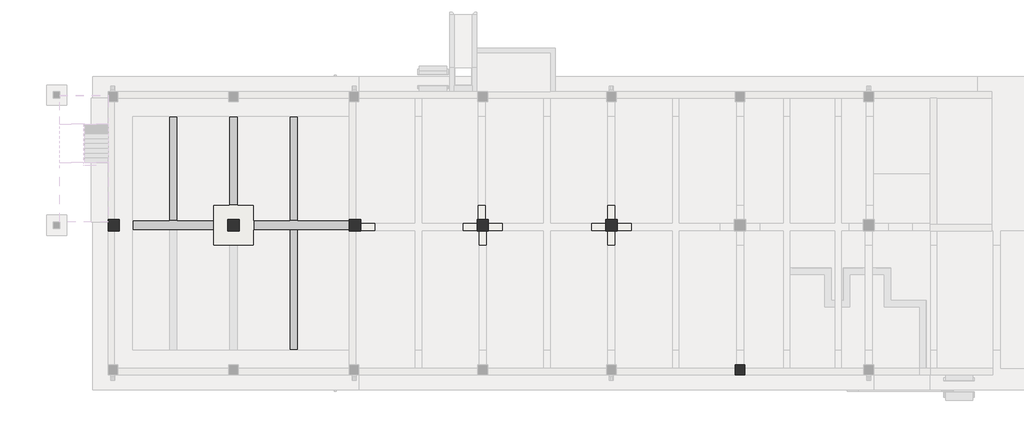
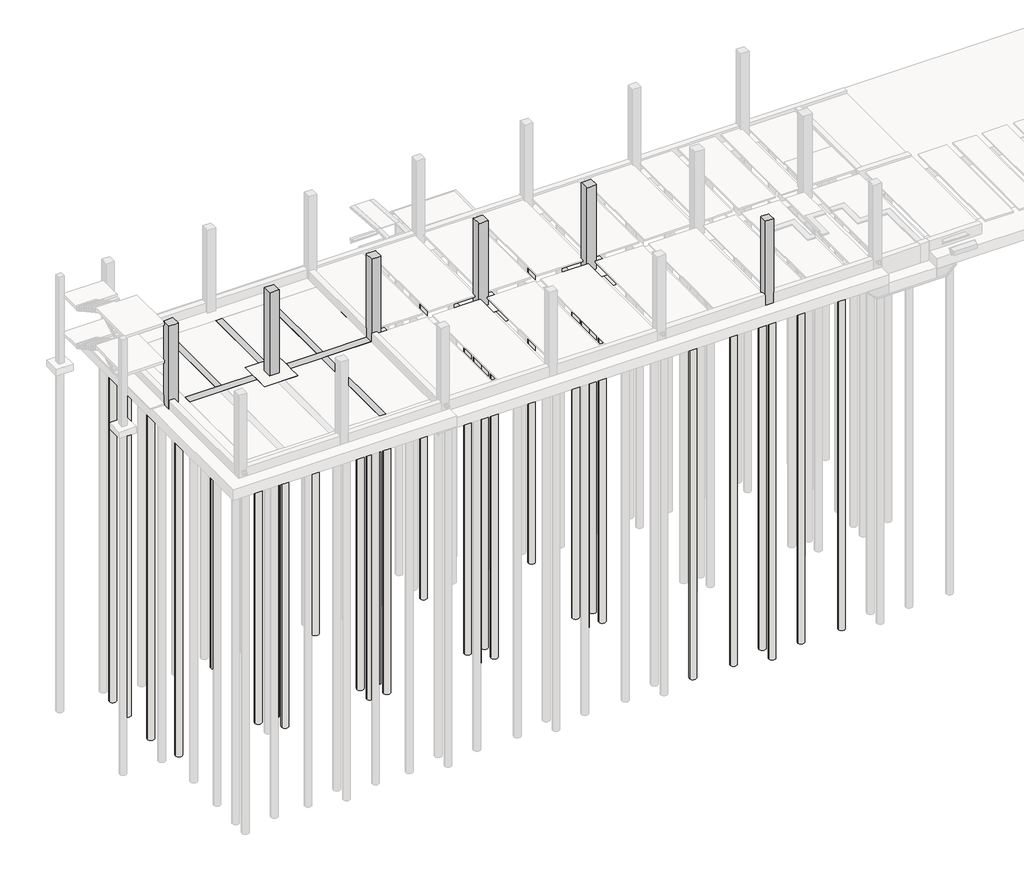
# One storey, part 4 of 7: 33 slabs, 8 beams, 6 columns.
"""IFC4 building model written with IfcOpenShell, lengths in millimetres."""

from ifc_helpers import new_model, si_unit, point, frame, frame_2d, origin, place, context, project, spatial, polyline, circle_curve, trimmed, segment, composite_curve, outline, extrude, faceted_brep, element, save

model = new_model("IFC4")

# Units and contexts
model_context = context("Model", 3, world=origin())
ifc_project = project(units=[si_unit("LENGTHUNIT", "METRE", prefix="MILLI")], contexts=[model_context])

# Site, building, storey
site = spatial("IfcSite", under=ifc_project)
building = spatial("IfcBuilding", under=site)
storey = spatial("IfcBuildingStorey", under=building, Name="H.P.P", Elevation=4500.0)

# Beams
placement = place(None, origin())
element("IfcBeam", 1, ObjectType="RC Beam_Rectangular : H_SB_AR S16_TG-UG_500x700_FB1A", at=placement, inside=storey, context=model_context, shape_type="Brep", body=[
    faceted_brep([(11000.0, -15750.0, 3400.0), (11500.0, -15750.0, 3400.0), (11500.0, -15750.0, 3840.0), (11500.0, -15750.0, 3950.0), (11500.0, -15750.0, 4100.0), (11000.0, -15750.0, 4100.0), (11000.0, -15750.0, 3950.0), (11000.0, -15750.0, 3840.0), (11500.0, -8299.9999999, 4100.0), (11000.0, -8299.9999999, 4100.0), (11500.0, -8299.9999999, 3950.0), (11500.0, -8299.9999999, 3400.0), (11500.0, -8299.9999999, 3840.0), (11000.0, -8299.9999999, 3400.0), (11000.0, -8299.9999999, 3950.0), (11000.0, -8299.9999999, 3840.0)], [[[0, 1, 2, 3, 4, 5, 6, 7]], [[5, 4, 8, 9]], [[10, 8, 4, 3, 2, 1, 11, 12]], [[1, 0, 13, 11]], [[9, 14, 15, 13, 0, 7, 6, 5]], [[9, 8, 10, 12, 11, 13, 15, 14]]]),
])
element("IfcBeam", 2, ObjectType="RC Beam_Rectangular : H_SB_AR S16_TG-UG_600x800_FG2", at=placement, inside=storey, context=model_context, shape_type="Brep", body=[
    faceted_brep([(6250.0000003, -7700.0, 4100.0), (6250.0000003, -8300.0, 4100.0), (6250.0000003, -8300.0, 3950.0), (6250.0000003, -8300.0, 3840.0), (6250.0000003, -8300.0, 3300.0), (6250.0000003, -7700.0, 3300.0), (6250.0000003, -7700.0, 3840.0), (6250.0000003, -7700.0, 3950.0), (1250.0000003, -7700.0, 3300.0), (1250.0000003, -8300.0, 3300.0), (1250.0000003, -8300.0, 3840.0), (1250.0000003, -8300.0, 3950.0), (1250.0000003, -8300.0, 4100.0), (1250.0000003, -7700.0, 4100.0), (1250.0000003, -7700.0, 3950.0), (1250.0000003, -7700.0, 3840.0), (4000.0, -7700.0, 4100.0), (3500.0, -7700.0, 4100.0), (3500.0, -8300.0, 4100.0), (4000.0, -8300.0, 4100.0)], [[[0, 1, 2, 3, 4, 5, 6, 7]], [[8, 9, 10, 11, 12, 13, 14, 15]], [[1, 0, 16, 17, 13, 12, 18, 19]], [[9, 4, 3, 2, 1, 19, 18, 12, 11, 10]], [[5, 4, 9, 8]], [[5, 8, 15, 14, 13, 17, 16, 0, 7, 6]]]),
])
element("IfcBeam", 3, ObjectType="RC Beam_Rectangular : H_SB_AR S16_TG-UG_600x800_FG2", at=placement, inside=storey, context=model_context, shape_type="Brep", body=[
    faceted_brep([(8750.0000003, -7699.9999999, 3300.0), (8750.0000003, -8299.9999999, 3300.0), (8750.0000003, -8299.9999999, 3840.0), (8750.0000003, -8299.9999999, 3950.0), (8750.0000003, -8299.9999999, 4100.0), (8750.0000003, -7699.9999999, 4100.0), (8750.0000003, -7699.9999999, 3950.0), (8750.0000003, -7699.9999999, 3840.0), (11000.0, -8299.9999999, 4100.0), (11500.0, -8299.9999999, 4100.0), (14700.0000001, -8299.9999999, 4100.0), (14700.0000001, -7699.9999999, 4100.0), (11500.0, -7699.9999999, 4100.0), (11000.0, -7699.9999999, 4100.0), (13800.0000001, -8299.9999999, 4000.0), (14700.0000001, -8299.9999999, 4000.0), (13800.0000001, -8299.9999999, 3300.0), (13800.0000001, -8299.9999999, 3840.0), (13800.0000001, -8299.9999999, 3950.0), (13800.0000001, -7699.9999999, 3300.0), (14700.0000001, -7699.9999999, 4000.0), (13800.0000001, -7699.9999999, 4000.0), (13800.0000001, -7699.9999999, 3950.0), (13800.0000001, -7699.9999999, 3840.0)], [[[0, 1, 2, 3, 4, 5, 6, 7]], [[5, 4, 8, 9, 10, 11, 12, 13]], [[14, 15, 10, 9, 8, 4, 3, 2, 1, 16, 17, 18]], [[1, 0, 19, 16]], [[20, 21, 22, 23, 19, 0, 7, 6, 5, 13, 12, 11]], [[14, 21, 20, 15]], [[21, 14, 18, 17, 16, 19, 23, 22]], [[11, 10, 15, 20]]]),
])
element("IfcBeam", 4, ObjectType="RC Beam_Rectangular : H_SB_AR S16_TG-UG_500x700_FG1", at=placement, inside=storey, context=model_context, shape_type="Brep", body=[
    faceted_brep([(14700.0, -15750.0, 4100.0), (14700.0, -15750.0, 3950.0), (14700.0, -15750.0, 3840.0), (14700.0, -15750.0, 3400.0), (15200.0, -15750.0, 3400.0), (15200.0, -15750.0, 4100.0), (15200.0, -8350.0, 4100.0), (15100.0, -8350.0, 4100.0), (14700.0, -8350.0, 4100.0), (15200.0, -9250.0, 3400.0), (15200.0, -9250.0, 4000.0), (15200.0, -8350.0, 4000.0), (14700.0, -9250.0, 3400.0), (14700.0, -8350.0, 4000.0), (14700.0, -9250.0, 4000.0), (14700.0, -9250.0, 3950.0), (14700.0, -9250.0, 3840.0)], [[[0, 1, 2, 3, 4, 5]], [[0, 5, 6, 7, 8]], [[5, 4, 9, 10, 11, 6]], [[4, 3, 12, 9]], [[3, 2, 1, 0, 8, 13, 14, 15, 16, 12]], [[10, 14, 13, 11]], [[14, 10, 9, 12, 16, 15]], [[8, 7, 6, 11, 13]]]),
])
element("IfcBeam", 5, ObjectType="RC Beam_Rectangular : H_SB_AR S16_TG-UG_500x700_FB1A", at=placement, inside=storey, context=model_context, shape_type="Brep", body=[
    faceted_brep([(4000.0, -1250.0000001, 3400.0), (3500.0, -1250.0000001, 3400.0), (3500.0, -1250.0000001, 3840.0), (3500.0, -1250.0000001, 3950.0), (3500.0, -1250.0000001, 4100.0), (4000.0, -1250.0000001, 4100.0), (4000.0, -1250.0000001, 3950.0), (4000.0, -1250.0000001, 3840.0), (3500.0, -7700.0, 4100.0), (4000.0, -7700.0, 4100.0), (4000.0, -7700.0, 3950.0), (4000.0, -7700.0, 3840.0), (4000.0, -7700.0, 3400.0), (3500.0, -7700.0, 3400.0), (3500.0, -7700.0, 3840.0), (3500.0, -7700.0, 3950.0)], [[[0, 1, 2, 3, 4, 5, 6, 7]], [[5, 4, 8, 9]], [[5, 9, 10, 11, 12, 0, 7, 6]], [[1, 0, 12, 13]], [[8, 4, 3, 2, 1, 13, 14, 15]], [[9, 8, 15, 14, 13, 12, 11, 10]]]),
])
element("IfcBeam", 6, ObjectType="RC Beam_Rectangular : H_SB_AR S16_TG-UG_500x700_FG1", at=placement, inside=storey, context=model_context, shape_type="Brep", body=[
    faceted_brep([(7750.0, -6750.0000001, 4100.0), (7250.0, -6750.0000001, 4100.0), (7250.0, -6750.0000001, 3950.0), (7250.0, -6750.0000001, 3840.0), (7250.0, -6750.0000001, 3400.0), (7750.0, -6750.0000001, 3400.0), (7750.0, -6750.0000001, 3840.0), (7750.0, -6750.0000001, 3950.0), (7750.0, -1250.0000001, 3400.0), (7250.0, -1250.0000001, 3400.0), (7250.0, -1250.0000001, 3840.0), (7250.0, -1250.0000001, 3950.0), (7250.0, -1250.0000001, 4100.0), (7750.0, -1250.0000001, 4100.0), (7750.0, -1250.0000001, 3950.0), (7750.0, -1250.0000001, 3840.0)], [[[0, 1, 2, 3, 4, 5, 6, 7]], [[8, 9, 10, 11, 12, 13, 14, 15]], [[1, 0, 13, 12]], [[13, 0, 7, 6, 5, 8, 15, 14]], [[5, 4, 9, 8]], [[1, 12, 11, 10, 9, 4, 3, 2]]]),
])
element("IfcBeam", 7, ObjectType="RC Beam_Rectangular : H_SB_AR S16_TG-UG_500x700_FB1A", at=placement, inside=storey, context=model_context, shape_type="Brep", body=[
    faceted_brep([(11500.0, -1250.0000001, 3400.0), (11000.0, -1250.0000001, 3400.0), (11000.0, -1250.0000001, 3840.0), (11000.0, -1250.0000001, 3950.0), (11000.0, -1250.0000001, 4100.0), (11500.0, -1250.0000001, 4100.0), (11500.0, -1250.0000001, 3950.0), (11500.0, -1250.0000001, 3840.0), (11000.0, -7699.9999999, 4100.0), (11500.0, -7699.9999999, 4100.0), (11500.0, -7699.9999999, 3950.0), (11500.0, -7699.9999999, 3840.0), (11500.0, -7699.9999999, 3400.0), (11000.0, -7699.9999999, 3400.0), (11000.0, -7699.9999999, 3840.0), (11000.0, -7699.9999999, 3950.0)], [[[0, 1, 2, 3, 4, 5, 6, 7]], [[5, 4, 8, 9]], [[5, 9, 10, 11, 12, 0, 7, 6]], [[1, 0, 12, 13]], [[8, 4, 3, 2, 1, 13, 14, 15]], [[9, 8, 15, 14, 13, 12, 11, 10]]]),
])
element("IfcBeam", 8, ObjectType="RC Beam_Rectangular : H_SB_AR S16_TG-UG_500x700_FG1", at=placement, inside=storey, context=model_context, shape_type="Brep", body=[
    faceted_brep([(14700.0, -1250.0000001, 3400.0), (14700.0, -1250.0000001, 3840.0), (14700.0, -1250.0000001, 3950.0), (14700.0, -1250.0000001, 4100.0), (15200.0, -1250.0000001, 4100.0), (15200.0, -1250.0000001, 3400.0), (14700.0, -7650.0, 4100.0), (15100.0, -7650.0, 4100.0), (15200.0, -7650.0, 4100.0), (15200.0, -7650.0, 4000.0), (15200.0, -6750.0, 4000.0), (15200.0, -6750.0, 3400.0), (14700.0, -6750.0, 3400.0), (14700.0, -6750.0, 3840.0), (14700.0, -6750.0, 3950.0), (14700.0, -6750.0, 4000.0), (14700.0, -7650.0, 4000.0)], [[[0, 1, 2, 3, 4, 5]], [[4, 3, 6, 7, 8]], [[5, 4, 8, 9, 10, 11]], [[0, 5, 11, 12]], [[3, 2, 1, 0, 12, 13, 14, 15, 16, 6]], [[15, 10, 9, 16]], [[10, 15, 14, 13, 12, 11]], [[8, 7, 6, 16, 9]]]),
])

# Columns
element("IfcColumn", 9, ObjectType="RC_Column_Rectangular : H_SC_AR S15_RC Col-AG_700x700_C1", at=placement, inside=storey, context=model_context, shape_type="Brep", body=[
    faceted_brep([(400.0, -7650.0, 4100.0), (400.0, -8350.0, 4100.0), (100.0, -8350.0, 4100.0), (-300.0, -8350.0, 4100.0), (-300.0, -7650.0, 4100.0), (100.0, -7650.0, 4100.0), (400.0, -7650.0, 10450.0), (400.0, -7700.0, 10450.0), (400.0, -7700.0, 10600.0), (400.0, -8300.0, 10600.0), (400.0, -8300.0, 10450.0), (400.0, -8350.0, 10450.0), (399.4974747, -8350.0, 10450.0), (399.4974747, -8350.0, 10600.0), (100.0, -8350.0, 10600.0), (-300.0, -8350.0, 10600.0), (-300.0, -8350.0, 9900.0), (-300.0, -8350.0, 4800.0), (-300.0, -7650.0, 10600.0), (-300.0, -7650.0, 9900.0), (-300.0, -7650.0, 4800.0), (100.0, -7650.0, 10600.0), (399.4974747, -7650.0, 10600.0), (399.4974747, -7650.0, 10450.0), (399.4974747, -8300.0, 10600.0), (399.4974747, -7700.0, 10600.0), (399.4974747, -7700.0, 10450.0), (399.4974747, -8300.0, 10450.0)], [[[0, 1, 2, 3, 4, 5]], [[1, 0, 6, 7, 8, 9, 10, 11]], [[3, 2, 1, 11, 12, 13, 14, 15, 16, 17]], [[4, 3, 17, 16, 15, 18, 19, 20]], [[0, 5, 4, 20, 19, 18, 21, 22, 23, 6]], [[18, 15, 14, 13, 24, 9, 8, 25, 22, 21]], [[23, 26, 7, 6]], [[26, 25, 8, 7]], [[26, 23, 22, 25]], [[12, 27, 24, 13]], [[24, 27, 10, 9]], [[27, 12, 11, 10]]]),
])
element("IfcColumn", 10, ObjectType="RC_Column_Rectangular : H_SC_AR S15_RC Col-AG_700x700_C1", at=placement, inside=storey, context=model_context, shape_type="Brep", body=[
    faceted_brep([(7850.0, -7650.0, 4100.0), (7850.0, -8350.0, 4100.0), (7150.0, -8350.0, 4100.0), (7150.0, -7650.0, 4100.0), (7850.0, -7650.0, 10450.0), (7850.0, -7650.0, 10600.0), (7850.0, -7700.0, 10600.0), (7850.0, -8300.0, 10600.0), (7850.0, -8350.0, 10600.0), (7850.0, -8350.0, 10450.0), (7750.0, -8350.0, 10600.0), (7250.0, -8350.0, 10600.0), (7150.0, -8350.0, 10600.0), (7150.0, -8350.0, 10450.0), (7150.0, -8300.0, 10600.0), (7150.0, -7700.0, 10600.0), (7150.0, -7650.0, 10600.0), (7150.0, -7650.0, 10450.0), (7250.0, -7650.0, 10600.0), (7750.0, -7650.0, 10600.0)], [[[0, 1, 2, 3]], [[1, 0, 4, 5, 6, 7, 8, 9]], [[2, 1, 9, 8, 10, 11, 12, 13]], [[3, 2, 13, 12, 14, 15, 16, 17]], [[0, 3, 17, 16, 18, 19, 5, 4]], [[18, 16, 15, 14, 12, 11, 10, 8, 7, 6, 5, 19]]]),
])
element("IfcColumn", 11, ObjectType="RC_Column_Rectangular : H_SC_AR S15_RC Col-AG_700x700_C1", at=placement, inside=storey, context=model_context, shape_type="Brep", body=[
    faceted_brep([(15400.0000001, -7650.0, 4000.0), (15400.0000001, -7850.0, 4000.0), (15400.0000001, -8350.0, 4000.0), (15200.0, -8350.0, 4000.0), (14700.0000001, -8350.0, 4000.0), (14700.0000001, -8299.9999999, 4000.0), (14700.0000001, -7699.9999999, 4000.0), (14700.0000001, -7650.0, 4000.0), (15200.0, -7650.0, 4000.0), (15400.0000001, -7650.0, 4650.0), (15400.0000001, -7650.0, 4800.0), (15400.0000001, -7650.0, 10450.0), (15400.0000001, -7650.0, 10600.0), (15400.0000001, -7700.0, 10600.0), (15400.0000001, -8300.0, 10600.0), (15400.0000001, -8350.0, 10600.0), (15400.0000001, -8350.0, 10450.0), (15400.0000001, -8350.0, 4800.0), (15400.0000001, -8350.0, 4650.0), (15200.0, -8350.0, 10600.0), (14700.0000001, -8350.0, 10600.0), (14700.0000001, -8350.0, 10450.0), (14700.0000001, -8350.0, 4800.0), (14700.0000001, -8350.0, 4100.0), (14700.0000001, -8300.0, 10600.0), (14700.0000001, -7700.0, 10600.0), (14700.0000001, -7650.0, 10600.0), (14700.0000001, -7650.0, 10450.0), (14700.0000001, -7650.0, 4800.0), (14700.0000001, -7650.0, 4100.0), (15200.0, -7650.0, 10600.0)], [[[0, 1, 2, 3, 4, 5, 6, 7, 8]], [[2, 1, 0, 9, 10, 11, 12, 13, 14, 15, 16, 17, 18]], [[4, 3, 2, 18, 17, 16, 15, 19, 20, 21, 22, 23]], [[7, 6, 5, 4, 23, 22, 21, 20, 24, 25, 26, 27, 28, 29]], [[0, 8, 7, 29, 28, 27, 26, 30, 12, 11, 10, 9]], [[13, 12, 30, 26, 25, 24, 20, 19, 15, 14]]]),
])
element("IfcColumn", 12, ObjectType="RC_Column_Rectangular : H_SC_AR S15_RC Col-AG_700x700_C1", at=placement, inside=storey, context=model_context, shape_type="Brep", body=[
    faceted_brep([(23350.0000003, -7650.0, 4000.0), (23350.0000003, -8350.0, 4000.0), (22650.0000003, -8350.0, 4000.0), (22650.0000003, -7650.0, 4000.0), (23350.0000003, -7650.0, 4650.0), (23350.0000003, -7650.0, 4800.0), (23350.0000003, -7650.0, 10450.0), (23350.0000003, -7650.0, 10600.0), (23350.0000003, -7700.0, 10600.0), (23350.0000003, -8300.0, 10600.0), (23350.0000003, -8350.0, 10600.0), (23350.0000003, -8350.0, 10450.0), (23350.0000003, -8350.0, 4800.0), (23350.0000003, -8350.0, 4650.0), (23200.0, -8350.0, 10600.0), (22700.0, -8350.0, 10600.0), (22650.0000003, -8350.0, 10600.0), (22650.0000003, -8350.0, 10450.0), (22650.0000003, -8350.0, 4800.0), (22650.0000003, -8350.0, 4650.0), (22650.0000003, -8300.0, 10600.0), (22650.0000003, -7700.0, 10600.0), (22650.0000003, -7650.0, 10600.0), (22650.0000003, -7650.0, 10450.0), (22650.0000003, -7650.0, 4800.0), (22650.0000003, -7650.0, 4650.0), (22700.0, -7650.0, 10600.0), (23200.0, -7650.0, 10600.0)], [[[0, 1, 2, 3]], [[1, 0, 4, 5, 6, 7, 8, 9, 10, 11, 12, 13]], [[2, 1, 13, 12, 11, 10, 14, 15, 16, 17, 18, 19]], [[3, 2, 19, 18, 17, 16, 20, 21, 22, 23, 24, 25]], [[0, 3, 25, 24, 23, 22, 26, 27, 7, 6, 5, 4]], [[8, 7, 27, 26, 22, 21, 20, 16, 15, 14, 10, 9]]]),
])
element("IfcColumn", 13, ObjectType="RC_Column_Rectangular : H_SC_AR S15_RC Col-AG_700x700_C1", at=placement, inside=storey, context=model_context, shape_type="Brep", body=[
    faceted_brep([(31350.0000002, -7650.0, 4000.0), (31350.0000002, -8350.0, 4000.0), (30650.0000002, -8350.0, 4000.0), (30650.0000002, -7650.0, 4000.0), (31350.0000002, -7650.0, 4650.0), (31350.0000002, -7650.0, 4800.0), (31350.0000002, -7650.0, 10450.0), (31350.0000002, -7650.0, 10600.0), (31350.0000002, -7700.0, 10600.0), (31350.0000002, -8300.0, 10600.0), (31350.0000002, -8350.0, 10600.0), (31350.0000002, -8350.0, 10450.0), (31350.0000002, -8350.0, 4800.0), (31350.0000002, -8350.0, 4650.0), (31249.9999998, -8350.0, 10600.0), (30750.0000002, -8350.0, 10600.0), (30650.0000002, -8350.0, 10600.0), (30650.0000002, -8350.0, 10450.0), (30650.0000002, -8350.0, 4800.0), (30650.0000002, -8350.0, 4650.0), (30650.0000002, -8300.0, 10600.0), (30650.0000002, -7700.0, 10600.0), (30650.0000002, -7650.0, 10600.0), (30650.0000002, -7650.0, 10450.0), (30650.0000002, -7650.0, 4800.0), (30650.0000002, -7650.0, 4650.0), (30750.0000002, -7650.0, 10600.0), (31249.9999998, -7650.0, 10600.0)], [[[0, 1, 2, 3]], [[1, 0, 4, 5, 6, 7, 8, 9, 10, 11, 12, 13]], [[2, 1, 13, 12, 11, 10, 14, 15, 16, 17, 18, 19]], [[3, 2, 19, 18, 17, 16, 20, 21, 22, 23, 24, 25]], [[0, 3, 25, 24, 23, 22, 26, 27, 7, 6, 5, 4]], [[8, 7, 27, 26, 22, 21, 20, 16, 15, 14, 10, 9]]]),
])
element("IfcColumn", 14, ObjectType="RC_Column_Rectangular : H_SC_AR S15_RC Col-AG_600x600_C2", at=placement, inside=storey, context=model_context, shape_type="Brep", body=[
    faceted_brep([(38700.0, -16700.0, 4000.0), (39300.0, -16700.0, 4000.0), (39300.0, -16900.0, 4000.0), (39300.0, -17300.0, 4000.0), (38700.0, -17300.0, 4000.0), (38700.0, -16900.0, 4000.0), (38700.0, -16700.0, 4650.0), (38700.0, -16700.0, 4800.0), (38700.0, -16700.0, 10450.0), (38700.0, -16700.0, 10600.0), (38750.0000002, -16700.0, 10600.0), (39249.9999998, -16700.0, 10600.0), (39300.0, -16700.0, 10600.0), (39300.0, -16700.0, 10450.0), (39300.0, -16700.0, 4800.0), (39300.0, -16700.0, 4650.0), (39300.0, -16900.0, 10600.0), (39300.0, -17300.0, 10600.0), (39300.0, -17300.0, 9800.0), (39300.0, -17300.0, 4800.0), (38700.0, -17300.0, 10600.0), (38700.0, -17300.0, 9800.0), (38700.0, -17300.0, 4800.0), (38700.0, -16900.0, 10600.0)], [[[0, 1, 2, 3, 4, 5]], [[1, 0, 6, 7, 8, 9, 10, 11, 12, 13, 14, 15]], [[3, 2, 1, 15, 14, 13, 12, 16, 17, 18, 19]], [[4, 3, 19, 18, 17, 20, 21, 22]], [[0, 5, 4, 22, 21, 20, 23, 9, 8, 7, 6]], [[20, 17, 16, 12, 11, 10, 9, 23]]]),
])

# Slabs
element("IfcSlab", 15, ObjectType="Foundation Rectangular (Non-Pile) : H_SF_AR S18_Ret Fdn_2500x2500xT1000_F1", at=placement, inside=storey, context=model_context, shape_type="Brep", body=[
    faceted_brep([(8750.0, -6750.0, 4100.0), (7750.0, -6750.0, 4100.0), (7250.0, -6750.0, 4100.0), (6250.0, -6750.0, 4100.0), (6250.0, -7700.0, 4100.0), (6250.0, -8300.0, 4100.0), (6250.0, -9250.0, 4100.0), (7250.0, -9250.0, 4100.0), (7750.0, -9250.0, 4100.0), (8750.0, -9250.0, 4100.0), (8750.0, -8299.9999999, 4100.0), (8750.0, -7699.9999999, 4100.0), (8750.0, -6750.0, 3100.0), (8750.0, -9250.0, 3100.0), (6250.0, -9250.0, 3100.0), (6250.0, -6750.0, 3100.0), (8750.0, -6750.0, 3840.0), (8750.0, -6750.0, 3790.0), (6250.0, -6750.0, 3790.0), (6250.0, -6750.0, 3840.0), (6250.0, -9250.0, 3790.0), (6250.0, -9250.0, 3840.0), (8750.0, -9250.0, 3790.0), (8750.0, -9250.0, 3840.0)], [[[0, 1, 2, 3, 4, 5, 6, 7, 8, 9, 10, 11]], [[12, 13, 14, 15]], [[3, 2, 1, 0, 16, 17, 12, 15, 18, 19]], [[6, 5, 4, 3, 19, 18, 15, 14, 20, 21]], [[9, 8, 7, 6, 21, 20, 14, 13, 22, 23]], [[0, 11, 10, 9, 23, 22, 13, 12, 17, 16]]]),
])
element("IfcSlab", 16, ObjectType="Foundation Rectangular (Non-Pile) : H_SF_AR S18_Ret Fdn_2500x2500xT1000_F1A", at=placement, inside=storey, context=model_context, shape_type="Brep", body=[
    faceted_brep([(16300.0000001, -6750.0, 4000.0), (15200.0, -6750.0, 4000.0), (14700.0, -6750.0, 4000.0), (13800.0000001, -6750.0, 4000.0), (13800.0000001, -7699.9999999, 4000.0), (13800.0000001, -8299.9999999, 4000.0), (13800.0000001, -9250.0, 4000.0), (14700.0, -9250.0, 4000.0), (15200.0, -9250.0, 4000.0), (16300.0000001, -9250.0, 4000.0), (16300.0000001, -6750.0, 3000.0), (16300.0000001, -9250.0, 3000.0), (13800.0000001, -9250.0, 3000.0), (13800.0000001, -6750.0, 3000.0), (13800.0000001, -6750.0, 3790.0), (13800.0000001, -6750.0, 3840.0), (13800.0000001, -6750.0, 3950.0), (13800.0000001, -9250.0, 3790.0), (13800.0000001, -9250.0, 3840.0), (13800.0000001, -9250.0, 3950.0)], [[[0, 1, 2, 3, 4, 5, 6, 7, 8, 9]], [[10, 11, 12, 13]], [[3, 2, 1, 0, 10, 13, 14, 15, 16]], [[6, 5, 4, 3, 16, 15, 14, 13, 12, 17, 18, 19]], [[9, 8, 7, 6, 19, 18, 17, 12, 11]], [[0, 9, 11, 10]]]),
])
element("IfcSlab", 17, ObjectType="Foundation Rectangular (Non-Pile) : H_SF_AR S18_Ret Fdn_2500x2500xT1000_F1A", at=placement, inside=storey, context=model_context, shape_type="SweptSolid", body=[
    extrude(outline(polyline([(24250.0000003, -6750.0), (24250.0000003, -9250.0), (21750.0000003, -9250.0), (21750.0000003, -6750.0), (24250.0000003, -6750.0)])), frame((0.0, 0.0, 3000.0), z_axis=(0.0, 0.0, 1.0), x_axis=(1.0, 0.0, 0.0)), (0.0, 0.0, 1.0), 1000.0),
])
element("IfcSlab", 18, ObjectType="Foundation Rectangular (Non-Pile) : H_SF_AR S18_Ret Fdn_2500x2500xT1000_F1A", at=placement, inside=storey, context=model_context, shape_type="SweptSolid", body=[
    extrude(outline(polyline([(32250.0000002, -6750.0), (32250.0000002, -9250.0), (29750.0000002, -9250.0), (29750.0000002, -6750.0), (32250.0000002, -6750.0)])), frame((0.0, 0.0, 3000.0), z_axis=(0.0, 0.0, 1.0), x_axis=(1.0, 0.0, 0.0)), (0.0, 0.0, 1.0), 1000.0),
])
element("IfcSlab", 19, ObjectType="PILE : H_FL_AR S19_Pile_D500_L26.9", at=placement, inside=storey, context=model_context, shape_type="SweptSolid", body=[
    extrude(outline(composite_curve([segment(trimmed(circle_curve(frame_2d((0.0, -625.0000002)), 250.0), [point((-250.0, -625.0000002))], [point((250.0, -625.0000002))], False, "CARTESIAN"), True, "CONTINUOUS"), segment(trimmed(circle_curve(frame_2d((0.0, -625.0000002)), 250.0), [point((250.0, -625.0000002))], [point((-250.0, -625.0000002))], False, "CARTESIAN"), True, "CONTINUOUS")], self_intersect=False)), frame((0.0, 0.0, -23500.0), z_axis=(0.0, 0.0, 1.0), x_axis=(1.0, 0.0, 0.0)), (0.0, 0.0, 1.0), 26750.0),
])
element("IfcSlab", 20, ObjectType="PILE : H_FL_AR S19_Pile_D500_L26.9", at=placement, inside=storey, context=model_context, shape_type="SweptSolid", body=[
    extrude(outline(composite_curve([segment(trimmed(circle_curve(frame_2d((0.0, -2500.0000003)), 250.0), [point((-250.0, -2500.0000003))], [point((250.0, -2500.0000003))], False, "CARTESIAN"), True, "CONTINUOUS"), segment(trimmed(circle_curve(frame_2d((0.0, -2500.0000003)), 250.0), [point((250.0, -2500.0000003))], [point((-250.0, -2500.0000003))], False, "CARTESIAN"), True, "CONTINUOUS")], self_intersect=False)), frame((0.0, 0.0, -23500.0), z_axis=(0.0, 0.0, 1.0), x_axis=(1.0, 0.0, 0.0)), (0.0, 0.0, 1.0), 26750.0),
])
element("IfcSlab", 21, ObjectType="PILE : H_FL_AR S19_Pile_D500_L26.9", at=placement, inside=storey, context=model_context, shape_type="SweptSolid", body=[
    extrude(outline(composite_curve([segment(trimmed(circle_curve(frame_2d((0.0, -5500.0000003)), 250.0), [point((-250.0, -5500.0000003))], [point((250.0, -5500.0000003))], False, "CARTESIAN"), True, "CONTINUOUS"), segment(trimmed(circle_curve(frame_2d((0.0, -5500.0000003)), 250.0), [point((250.0, -5500.0000003))], [point((-250.0, -5500.0000003))], False, "CARTESIAN"), True, "CONTINUOUS")], self_intersect=False)), frame((0.0, 0.0, -23500.0), z_axis=(0.0, 0.0, 1.0), x_axis=(1.0, 0.0, 0.0)), (0.0, 0.0, 1.0), 26750.0),
])
element("IfcSlab", 22, ObjectType="PILE : H_FL_AR S19_Pile_D500_L26.9", at=placement, inside=storey, context=model_context, shape_type="SweptSolid", body=[
    extrude(outline(composite_curve([segment(trimmed(circle_curve(frame_2d((624.9999999, -8000.0)), 250.0), [point((374.9999999, -8000.0))], [point((874.9999999, -8000.0))], False, "CARTESIAN"), True, "CONTINUOUS"), segment(trimmed(circle_curve(frame_2d((624.9999999, -8000.0)), 250.0), [point((874.9999999, -8000.0))], [point((374.9999999, -8000.0))], False, "CARTESIAN"), True, "CONTINUOUS")], self_intersect=False)), frame((0.0, 0.0, -23500.0), z_axis=(0.0, 0.0, 1.0), x_axis=(1.0, 0.0, 0.0)), (0.0, 0.0, 1.0), 26750.0),
])
element("IfcSlab", 23, ObjectType="PILE : H_FL_AR S19_Pile_D500_L26.9", at=placement, inside=storey, context=model_context, shape_type="SweptSolid", body=[
    extrude(outline(composite_curve([segment(trimmed(circle_curve(frame_2d((7500.0, -625.0000001)), 250.0), [point((7250.0, -625.0000001))], [point((7750.0, -625.0000001))], False, "CARTESIAN"), True, "CONTINUOUS"), segment(trimmed(circle_curve(frame_2d((7500.0, -625.0000001)), 250.0), [point((7750.0, -625.0000001))], [point((7250.0, -625.0000001))], False, "CARTESIAN"), True, "CONTINUOUS")], self_intersect=False)), frame((0.0, 0.0, -23500.0), z_axis=(0.0, 0.0, 1.0), x_axis=(1.0, 0.0, 0.0)), (0.0, 0.0, 1.0), 26750.0),
])
element("IfcSlab", 24, ObjectType="PILE : H_FL_AR S19_Pile_D500_L26.8", at=placement, inside=storey, context=model_context, shape_type="SweptSolid", body=[
    extrude(outline(composite_curve([segment(trimmed(circle_curve(frame_2d((14999.9999999, -625.0000002)), 250.0), [point((15249.9999999, -625.0000002))], [point((14749.9999999, -625.0000002))], False, "CARTESIAN"), True, "CONTINUOUS"), segment(trimmed(circle_curve(frame_2d((14999.9999999, -625.0000002)), 250.0), [point((14749.9999999, -625.0000002))], [point((15249.9999999, -625.0000002))], False, "CARTESIAN"), True, "CONTINUOUS")], self_intersect=False)), frame((0.0, 0.0, 3200.0), z_axis=(0.0, 0.0, 1.0), x_axis=(1.0, 0.0, 0.0)), (0.0, 0.0, 1.0), 100.0),
    extrude(outline(composite_curve([segment(trimmed(circle_curve(frame_2d((14999.9999999, -625.0000002)), 250.0), [point((14749.9999999, -625.0000002))], [point((15249.9999999, -625.0000002))], False, "CARTESIAN"), True, "CONTINUOUS"), segment(trimmed(circle_curve(frame_2d((14999.9999999, -625.0000002)), 250.0), [point((15249.9999999, -625.0000002))], [point((14749.9999999, -625.0000002))], False, "CARTESIAN"), True, "CONTINUOUS")], self_intersect=False)), frame((0.0, 0.0, -23500.0), z_axis=(0.0, 0.0, 1.0), x_axis=(1.0, 0.0, 0.0)), (0.0, 0.0, 1.0), 26650.0),
])
element("IfcSlab", 25, ObjectType="PILE : H_FL_AR S19_Pile_D500_L26.8", at=placement, inside=storey, context=model_context, shape_type="SweptSolid", body=[
    extrude(outline(composite_curve([segment(trimmed(circle_curve(frame_2d((22999.9999996, -625.0000002)), 250.0), [point((22749.9999996, -625.0000002))], [point((23249.9999996, -625.0000002))], False, "CARTESIAN"), True, "CONTINUOUS"), segment(trimmed(circle_curve(frame_2d((22999.9999996, -625.0000002)), 250.0), [point((23249.9999996, -625.0000002))], [point((22749.9999996, -625.0000002))], False, "CARTESIAN"), True, "CONTINUOUS")], self_intersect=False)), frame((0.0, 0.0, -23500.0), z_axis=(0.0, 0.0, 1.0), x_axis=(1.0, 0.0, 0.0)), (0.0, 0.0, 1.0), 26650.0),
])
element("IfcSlab", 26, ObjectType="PILE : H_FL_AR S19_Pile_D500_L26.8", at=placement, inside=storey, context=model_context, shape_type="SweptSolid", body=[
    extrude(outline(composite_curve([segment(trimmed(circle_curve(frame_2d((31000.0, -625.0000001)), 250.0), [point((30750.0, -625.0000001))], [point((31250.0, -625.0000001))], False, "CARTESIAN"), True, "CONTINUOUS"), segment(trimmed(circle_curve(frame_2d((31000.0, -625.0000001)), 250.0), [point((31250.0, -625.0000001))], [point((30750.0, -625.0000001))], False, "CARTESIAN"), True, "CONTINUOUS")], self_intersect=False)), frame((0.0, 0.0, -23500.0), z_axis=(0.0, 0.0, 1.0), x_axis=(1.0, 0.0, 0.0)), (0.0, 0.0, 1.0), 26650.0),
])
element("IfcSlab", 27, ObjectType="PILE : H_FL_AR S19_Pile_D500_L26.7", at=placement, inside=storey, context=model_context, shape_type="SweptSolid", body=[
    extrude(outline(composite_curve([segment(trimmed(circle_curve(frame_2d((6875.0000004, -7374.9999999)), 250.0), [point((6625.0000004, -7374.9999999))], [point((7125.0000004, -7374.9999999))], False, "CARTESIAN"), True, "CONTINUOUS"), segment(trimmed(circle_curve(frame_2d((6875.0000004, -7374.9999999)), 250.0), [point((7125.0000004, -7374.9999999))], [point((6625.0000004, -7374.9999999))], False, "CARTESIAN"), True, "CONTINUOUS")], self_intersect=False)), frame((0.0, 0.0, -23500.0), z_axis=(0.0, 0.0, 1.0), x_axis=(1.0, 0.0, 0.0)), (0.0, 0.0, 1.0), 26550.0),
])
element("IfcSlab", 28, ObjectType="PILE : H_FL_AR S19_Pile_D500_L26.7", at=placement, inside=storey, context=model_context, shape_type="SweptSolid", body=[
    extrude(outline(composite_curve([segment(trimmed(circle_curve(frame_2d((8125.0000004, -7374.9999999)), 250.0), [point((7875.0000004, -7374.9999999))], [point((8375.0000004, -7374.9999999))], False, "CARTESIAN"), True, "CONTINUOUS"), segment(trimmed(circle_curve(frame_2d((8125.0000004, -7374.9999999)), 250.0), [point((8375.0000004, -7374.9999999))], [point((7875.0000004, -7374.9999999))], False, "CARTESIAN"), True, "CONTINUOUS")], self_intersect=False)), frame((0.0, 0.0, -23500.0), z_axis=(0.0, 0.0, 1.0), x_axis=(1.0, 0.0, 0.0)), (0.0, 0.0, 1.0), 26550.0),
])
element("IfcSlab", 29, ObjectType="PILE : H_FL_AR S19_Pile_D500_L26.7", at=placement, inside=storey, context=model_context, shape_type="SweptSolid", body=[
    extrude(outline(composite_curve([segment(trimmed(circle_curve(frame_2d((8125.0000004, -8624.9999999)), 250.0), [point((7875.0000004, -8624.9999999))], [point((8375.0000004, -8624.9999999))], False, "CARTESIAN"), True, "CONTINUOUS"), segment(trimmed(circle_curve(frame_2d((8125.0000004, -8624.9999999)), 250.0), [point((8375.0000004, -8624.9999999))], [point((7875.0000004, -8624.9999999))], False, "CARTESIAN"), True, "CONTINUOUS")], self_intersect=False)), frame((0.0, 0.0, -23500.0), z_axis=(0.0, 0.0, 1.0), x_axis=(1.0, 0.0, 0.0)), (0.0, 0.0, 1.0), 26550.0),
])
element("IfcSlab", 30, ObjectType="PILE : H_FL_AR S19_Pile_D500_L26.6", at=placement, inside=storey, context=model_context, shape_type="SweptSolid", body=[
    extrude(outline(composite_curve([segment(trimmed(circle_curve(frame_2d((14425.0000004, -7374.9999999)), 250.0), [point((14175.0000004, -7374.9999999))], [point((14675.0000004, -7374.9999999))], False, "CARTESIAN"), True, "CONTINUOUS"), segment(trimmed(circle_curve(frame_2d((14425.0000004, -7374.9999999)), 250.0), [point((14675.0000004, -7374.9999999))], [point((14175.0000004, -7374.9999999))], False, "CARTESIAN"), True, "CONTINUOUS")], self_intersect=False)), frame((0.0, 0.0, -23500.0), z_axis=(0.0, 0.0, 1.0), x_axis=(1.0, 0.0, 0.0)), (0.0, 0.0, 1.0), 26450.0),
])
element("IfcSlab", 31, ObjectType="PILE : H_FL_AR S19_Pile_D500_L26.6", at=placement, inside=storey, context=model_context, shape_type="SweptSolid", body=[
    extrude(outline(composite_curve([segment(trimmed(circle_curve(frame_2d((15675.0000004, -7374.9999999)), 250.0), [point((15425.0000004, -7374.9999999))], [point((15925.0000004, -7374.9999999))], False, "CARTESIAN"), True, "CONTINUOUS"), segment(trimmed(circle_curve(frame_2d((15675.0000004, -7374.9999999)), 250.0), [point((15925.0000004, -7374.9999999))], [point((15425.0000004, -7374.9999999))], False, "CARTESIAN"), True, "CONTINUOUS")], self_intersect=False)), frame((0.0, 0.0, -23500.0), z_axis=(0.0, 0.0, 1.0), x_axis=(1.0, 0.0, 0.0)), (0.0, 0.0, 1.0), 26450.0),
])
element("IfcSlab", 32, ObjectType="PILE : H_FL_AR S19_Pile_D500_L26.6", at=placement, inside=storey, context=model_context, shape_type="SweptSolid", body=[
    extrude(outline(composite_curve([segment(trimmed(circle_curve(frame_2d((14425.0000004, -8624.9999999)), 250.0), [point((14175.0000004, -8624.9999999))], [point((14675.0000004, -8624.9999999))], False, "CARTESIAN"), True, "CONTINUOUS"), segment(trimmed(circle_curve(frame_2d((14425.0000004, -8624.9999999)), 250.0), [point((14675.0000004, -8624.9999999))], [point((14175.0000004, -8624.9999999))], False, "CARTESIAN"), True, "CONTINUOUS")], self_intersect=False)), frame((0.0, 0.0, -23500.0), z_axis=(0.0, 0.0, 1.0), x_axis=(1.0, 0.0, 0.0)), (0.0, 0.0, 1.0), 26450.0),
])
element("IfcSlab", 33, ObjectType="PILE : H_FL_AR S19_Pile_D500_L26.6", at=placement, inside=storey, context=model_context, shape_type="SweptSolid", body=[
    extrude(outline(composite_curve([segment(trimmed(circle_curve(frame_2d((15675.0000004, -8624.9999999)), 250.0), [point((15425.0000004, -8624.9999999))], [point((15925.0000004, -8624.9999999))], False, "CARTESIAN"), True, "CONTINUOUS"), segment(trimmed(circle_curve(frame_2d((15675.0000004, -8624.9999999)), 250.0), [point((15925.0000004, -8624.9999999))], [point((15425.0000004, -8624.9999999))], False, "CARTESIAN"), True, "CONTINUOUS")], self_intersect=False)), frame((0.0, 0.0, -23500.0), z_axis=(0.0, 0.0, 1.0), x_axis=(1.0, 0.0, 0.0)), (0.0, 0.0, 1.0), 26450.0),
])
element("IfcSlab", 34, ObjectType="PILE : H_FL_AR S19_Pile_D500_L26.6", at=placement, inside=storey, context=model_context, shape_type="SweptSolid", body=[
    extrude(outline(composite_curve([segment(trimmed(circle_curve(frame_2d((22375.0000006, -7374.9999999)), 250.0), [point((22125.0000006, -7374.9999999))], [point((22625.0000006, -7374.9999999))], False, "CARTESIAN"), True, "CONTINUOUS"), segment(trimmed(circle_curve(frame_2d((22375.0000006, -7374.9999999)), 250.0), [point((22625.0000006, -7374.9999999))], [point((22125.0000006, -7374.9999999))], False, "CARTESIAN"), True, "CONTINUOUS")], self_intersect=False)), frame((0.0, 0.0, -23500.0), z_axis=(0.0, 0.0, 1.0), x_axis=(1.0, 0.0, 0.0)), (0.0, 0.0, 1.0), 26450.0),
])
element("IfcSlab", 35, ObjectType="PILE : H_FL_AR S19_Pile_D500_L26.6", at=placement, inside=storey, context=model_context, shape_type="SweptSolid", body=[
    extrude(outline(composite_curve([segment(trimmed(circle_curve(frame_2d((23625.0000006, -7374.9999999)), 250.0), [point((23375.0000006, -7374.9999999))], [point((23875.0000006, -7374.9999999))], False, "CARTESIAN"), True, "CONTINUOUS"), segment(trimmed(circle_curve(frame_2d((23625.0000006, -7374.9999999)), 250.0), [point((23875.0000006, -7374.9999999))], [point((23375.0000006, -7374.9999999))], False, "CARTESIAN"), True, "CONTINUOUS")], self_intersect=False)), frame((0.0, 0.0, -23500.0), z_axis=(0.0, 0.0, 1.0), x_axis=(1.0, 0.0, 0.0)), (0.0, 0.0, 1.0), 26450.0),
])
element("IfcSlab", 36, ObjectType="PILE : H_FL_AR S19_Pile_D500_L26.6", at=placement, inside=storey, context=model_context, shape_type="SweptSolid", body=[
    extrude(outline(composite_curve([segment(trimmed(circle_curve(frame_2d((22375.0000006, -8624.9999999)), 250.0), [point((22125.0000006, -8624.9999999))], [point((22625.0000006, -8624.9999999))], False, "CARTESIAN"), True, "CONTINUOUS"), segment(trimmed(circle_curve(frame_2d((22375.0000006, -8624.9999999)), 250.0), [point((22625.0000006, -8624.9999999))], [point((22125.0000006, -8624.9999999))], False, "CARTESIAN"), True, "CONTINUOUS")], self_intersect=False)), frame((0.0, 0.0, -23500.0), z_axis=(0.0, 0.0, 1.0), x_axis=(1.0, 0.0, 0.0)), (0.0, 0.0, 1.0), 26450.0),
])
element("IfcSlab", 37, ObjectType="PILE : H_FL_AR S19_Pile_D500_L26.6", at=placement, inside=storey, context=model_context, shape_type="SweptSolid", body=[
    extrude(outline(composite_curve([segment(trimmed(circle_curve(frame_2d((23625.0000006, -8624.9999999)), 250.0), [point((23375.0000006, -8624.9999999))], [point((23875.0000006, -8624.9999999))], False, "CARTESIAN"), True, "CONTINUOUS"), segment(trimmed(circle_curve(frame_2d((23625.0000006, -8624.9999999)), 250.0), [point((23875.0000006, -8624.9999999))], [point((23375.0000006, -8624.9999999))], False, "CARTESIAN"), True, "CONTINUOUS")], self_intersect=False)), frame((0.0, 0.0, -23500.0), z_axis=(0.0, 0.0, 1.0), x_axis=(1.0, 0.0, 0.0)), (0.0, 0.0, 1.0), 26450.0),
])
element("IfcSlab", 38, ObjectType="PILE : H_FL_AR S19_Pile_D500_L26.6", at=placement, inside=storey, context=model_context, shape_type="SweptSolid", body=[
    extrude(outline(composite_curve([segment(trimmed(circle_curve(frame_2d((30375.0000004, -7374.9999999)), 250.0), [point((30125.0000004, -7374.9999999))], [point((30625.0000004, -7374.9999999))], False, "CARTESIAN"), True, "CONTINUOUS"), segment(trimmed(circle_curve(frame_2d((30375.0000004, -7374.9999999)), 250.0), [point((30625.0000004, -7374.9999999))], [point((30125.0000004, -7374.9999999))], False, "CARTESIAN"), True, "CONTINUOUS")], self_intersect=False)), frame((0.0, 0.0, -23500.0), z_axis=(0.0, 0.0, 1.0), x_axis=(1.0, 0.0, 0.0)), (0.0, 0.0, 1.0), 26450.0),
])
element("IfcSlab", 39, ObjectType="PILE : H_FL_AR S19_Pile_D500_L26.6", at=placement, inside=storey, context=model_context, shape_type="SweptSolid", body=[
    extrude(outline(composite_curve([segment(trimmed(circle_curve(frame_2d((31625.0000004, -7374.9999999)), 250.0), [point((31375.0000004, -7374.9999999))], [point((31875.0000004, -7374.9999999))], False, "CARTESIAN"), True, "CONTINUOUS"), segment(trimmed(circle_curve(frame_2d((31625.0000004, -7374.9999999)), 250.0), [point((31875.0000004, -7374.9999999))], [point((31375.0000004, -7374.9999999))], False, "CARTESIAN"), True, "CONTINUOUS")], self_intersect=False)), frame((0.0, 0.0, -23500.0), z_axis=(0.0, 0.0, 1.0), x_axis=(1.0, 0.0, 0.0)), (0.0, 0.0, 1.0), 26450.0),
])
element("IfcSlab", 40, ObjectType="PILE : H_FL_AR S19_Pile_D500_L26.6", at=placement, inside=storey, context=model_context, shape_type="SweptSolid", body=[
    extrude(outline(composite_curve([segment(trimmed(circle_curve(frame_2d((30375.0000004, -8624.9999999)), 250.0), [point((30125.0000004, -8624.9999999))], [point((30625.0000004, -8624.9999999))], False, "CARTESIAN"), True, "CONTINUOUS"), segment(trimmed(circle_curve(frame_2d((30375.0000004, -8624.9999999)), 250.0), [point((30625.0000004, -8624.9999999))], [point((30125.0000004, -8624.9999999))], False, "CARTESIAN"), True, "CONTINUOUS")], self_intersect=False)), frame((0.0, 0.0, -23500.0), z_axis=(0.0, 0.0, 1.0), x_axis=(1.0, 0.0, 0.0)), (0.0, 0.0, 1.0), 26450.0),
])
element("IfcSlab", 41, ObjectType="PILE : H_FL_AR S19_Pile_D500_L26.6", at=placement, inside=storey, context=model_context, shape_type="SweptSolid", body=[
    extrude(outline(composite_curve([segment(trimmed(circle_curve(frame_2d((31625.0000004, -8624.9999999)), 250.0), [point((31375.0000004, -8624.9999999))], [point((31875.0000004, -8624.9999999))], False, "CARTESIAN"), True, "CONTINUOUS"), segment(trimmed(circle_curve(frame_2d((31625.0000004, -8624.9999999)), 250.0), [point((31875.0000004, -8624.9999999))], [point((31375.0000004, -8624.9999999))], False, "CARTESIAN"), True, "CONTINUOUS")], self_intersect=False)), frame((0.0, 0.0, -23500.0), z_axis=(0.0, 0.0, 1.0), x_axis=(1.0, 0.0, 0.0)), (0.0, 0.0, 1.0), 26450.0),
])
element("IfcSlab", 42, ObjectType="PILE : H_FL_AR S19_Pile_D500_L26.8", at=placement, inside=storey, context=model_context, shape_type="SweptSolid", body=[
    extrude(outline(composite_curve([segment(trimmed(circle_curve(frame_2d((33500.0000012, -17000.0)), 250.0), [point((33250.0000012, -17000.0))], [point((33750.0000012, -17000.0))], False, "CARTESIAN"), True, "CONTINUOUS"), segment(trimmed(circle_curve(frame_2d((33500.0000012, -17000.0)), 250.0), [point((33750.0000012, -17000.0))], [point((33250.0000012, -17000.0))], False, "CARTESIAN"), True, "CONTINUOUS")], self_intersect=False)), frame((0.0, 0.0, -23500.0), z_axis=(0.0, 0.0, 1.0), x_axis=(1.0, 0.0, 0.0)), (0.0, 0.0, 1.0), 26650.0),
])
element("IfcSlab", 43, ObjectType="PILE : H_FL_AR S19_Pile_D500_L26.8", at=placement, inside=storey, context=model_context, shape_type="SweptSolid", body=[
    extrude(outline(composite_curve([segment(trimmed(circle_curve(frame_2d((36500.0000003, -17000.0)), 250.0), [point((36250.0000003, -17000.0))], [point((36750.0000003, -17000.0))], False, "CARTESIAN"), True, "CONTINUOUS"), segment(trimmed(circle_curve(frame_2d((36500.0000003, -17000.0)), 250.0), [point((36750.0000003, -17000.0))], [point((36250.0000003, -17000.0))], False, "CARTESIAN"), True, "CONTINUOUS")], self_intersect=False)), frame((0.0, 0.0, -23500.0), z_axis=(0.0, 0.0, 1.0), x_axis=(1.0, 0.0, 0.0)), (0.0, 0.0, 1.0), 26650.0),
])
element("IfcSlab", 44, ObjectType="PILE : H_FL_AR S19_Pile_D500_L26.8", at=placement, inside=storey, context=model_context, shape_type="SweptSolid", body=[
    extrude(outline(composite_curve([segment(trimmed(circle_curve(frame_2d((39000.0, -16375.0000002)), 250.0), [point((38750.0, -16375.0000002))], [point((39250.0, -16375.0000002))], False, "CARTESIAN"), True, "CONTINUOUS"), segment(trimmed(circle_curve(frame_2d((39000.0, -16375.0000002)), 250.0), [point((39250.0, -16375.0000002))], [point((38750.0, -16375.0000002))], False, "CARTESIAN"), True, "CONTINUOUS")], self_intersect=False)), frame((0.0, 0.0, -23500.0), z_axis=(0.0, 0.0, 1.0), x_axis=(1.0, 0.0, 0.0)), (0.0, 0.0, 1.0), 26650.0),
])
element("IfcSlab", 45, ObjectType="PILE : H_FL_AR S19_Pile_D500_L26.8", at=placement, inside=storey, context=model_context, shape_type="SweptSolid", body=[
    extrude(outline(composite_curve([segment(trimmed(circle_curve(frame_2d((39000.0, -17624.9999997)), 250.0), [point((38750.0, -17624.9999997))], [point((39250.0, -17624.9999997))], False, "CARTESIAN"), True, "CONTINUOUS"), segment(trimmed(circle_curve(frame_2d((39000.0, -17624.9999997)), 250.0), [point((39250.0, -17624.9999997))], [point((38750.0, -17624.9999997))], False, "CARTESIAN"), True, "CONTINUOUS")], self_intersect=False)), frame((0.0, 0.0, -23500.0), z_axis=(0.0, 0.0, 1.0), x_axis=(1.0, 0.0, 0.0)), (0.0, 0.0, 1.0), 26650.0),
])
element("IfcSlab", 46, ObjectType="PILE : H_FL_AR S19_Pile_D500_L26.8", at=placement, inside=storey, context=model_context, shape_type="SweptSolid", body=[
    extrude(outline(composite_curve([segment(trimmed(circle_curve(frame_2d((41500.0000012, -17000.0)), 250.0), [point((41250.0000012, -17000.0))], [point((41750.0000012, -17000.0))], False, "CARTESIAN"), True, "CONTINUOUS"), segment(trimmed(circle_curve(frame_2d((41500.0000012, -17000.0)), 250.0), [point((41750.0000012, -17000.0))], [point((41250.0000012, -17000.0))], False, "CARTESIAN"), True, "CONTINUOUS")], self_intersect=False)), frame((0.0, 0.0, -23500.0), z_axis=(0.0, 0.0, 1.0), x_axis=(1.0, 0.0, 0.0)), (0.0, 0.0, 1.0), 26650.0),
])
element("IfcSlab", 47, ObjectType="PILE : H_FL_AR S19_Pile_D500_L26.8", at=placement, inside=storey, context=model_context, shape_type="SweptSolid", body=[
    extrude(outline(composite_curve([segment(trimmed(circle_curve(frame_2d((44500.0000002, -17000.0)), 250.0), [point((44250.0000002, -17000.0))], [point((44750.0000002, -17000.0))], False, "CARTESIAN"), True, "CONTINUOUS"), segment(trimmed(circle_curve(frame_2d((44500.0000002, -17000.0)), 250.0), [point((44750.0000002, -17000.0))], [point((44250.0000002, -17000.0))], False, "CARTESIAN"), True, "CONTINUOUS")], self_intersect=False)), frame((0.0, 0.0, -23500.0), z_axis=(0.0, 0.0, 1.0), x_axis=(1.0, 0.0, 0.0)), (0.0, 0.0, 1.0), 26650.0),
])

save(model, "model.ifc")

# Revit data of these elements
# Type "RC Beam_Rectangular : H_SB_AR S16_TG-UG_500x700_FB1A"
#   Type Comments = "CV-UG"
#   중앙부 하부근 = ""
#   중앙부 상부근 = ""
#   중앙부 보조근 = ""
#   중앙부 늑근 = ""
#   외단부 하부근 = ""
#   외단부 상부근 = ""
#   외단부 보조근 = ""
#   외단부 늑근 = ""
#   부호 = "TG3"
#   내단부 하부근 = ""
#   내단부 상부근 = ""
#   내단부 보조근 = ""
#   내단부 늑근 = ""
#   ALL 하부근 = "3-D20"
#   ALL 상부근 = "3-D20"
#   ALL 보조근 = ""
#   ALL 늑근 = "2-D10 @120"
#   H_Rebar Ratio = 0.14
#   Width = 500 mm
#   Height = 700 mm
#   Length [instance default] = 1524 mm
#   b = 500 mm
#   h = 700 mm
#   hec_material3 [instance default] = none
#   hec_material2 [instance default] = none
#   hec_material1 [instance default] = none
#   Structural Material [instance default] = none
#   Assembly Code = ""
# Type "RC Beam_Rectangular : H_SB_AR S16_TG-UG_600x800_FG2"
#   Type Comments = "CV-UG"
#   중앙부 하부근 = ""
#   중앙부 상부근 = ""
#   중앙부 보조근 = ""
#   중앙부 늑근 = ""
#   외단부 하부근 = ""
#   외단부 상부근 = ""
#   외단부 보조근 = ""
#   외단부 늑근 = ""
#   부호 = "TG3"
#   내단부 하부근 = ""
#   내단부 상부근 = ""
#   내단부 보조근 = ""
#   내단부 늑근 = ""
#   ALL 하부근 = "3-D20"
#   ALL 상부근 = "3-D20"
#   ALL 보조근 = ""
#   ALL 늑근 = "2-D10 @120"
#   H_Rebar Ratio = 0.14
#   Width = 600 mm
#   Height = 800 mm
#   Length [instance default] = 1524 mm
#   b = 600 mm
#   h = 800 mm
#   hec_material3 [instance default] = none
#   hec_material2 [instance default] = none
#   hec_material1 [instance default] = none
#   Structural Material [instance default] = none
#   Assembly Code = ""
# Type "RC Beam_Rectangular : H_SB_AR S16_TG-UG_500x700_FG1"
#   Type Comments = "CV-UG"
#   중앙부 하부근 = ""
#   중앙부 상부근 = ""
#   중앙부 보조근 = ""
#   중앙부 늑근 = ""
#   외단부 하부근 = ""
#   외단부 상부근 = ""
#   외단부 보조근 = ""
#   외단부 늑근 = ""
#   부호 = "TG3"
#   내단부 하부근 = ""
#   내단부 상부근 = ""
#   내단부 보조근 = ""
#   내단부 늑근 = ""
#   ALL 하부근 = "3-D20"
#   ALL 상부근 = "3-D20"
#   ALL 보조근 = ""
#   ALL 늑근 = "2-D10 @120"
#   H_Rebar Ratio = 0.14
#   Width = 500 mm
#   Height = 700 mm
#   Length [instance default] = 1524 mm
#   b = 500 mm
#   h = 700 mm
#   hec_material3 [instance default] = none
#   hec_material2 [instance default] = none
#   hec_material1 [instance default] = none
#   Structural Material [instance default] = none
#   Assembly Code = ""
# Type "RC_Column_Rectangular : H_SC_AR S15_RC Col-AG_700x700_C1"
#   Type Comments = "CV-AG"
#   H_Rebar Ratio = 0.3
#   Width = 700 mm
#   Length = 700 mm
#   hec_material3 [instance default] = none
#   hec_material2 [instance default] = none
#   hec_material1 [instance default] = none
#   Structural Material [instance default] = none
#   Description = (empty or 0)
# Type "RC_Column_Rectangular : H_SC_AR S15_RC Col-AG_600x600_C2"
#   Type Comments = "CV-AG"
#   H_Rebar Ratio = 0.3
#   Width = 600 mm
#   Length = 600 mm
#   hec_material3 [instance default] = none
#   hec_material2 [instance default] = none
#   hec_material1 [instance default] = none
#   Structural Material [instance default] = none
#   Description = (empty or 0)
# Type "Foundation Rectangular (Non-Pile) : H_SF_AR S18_Ret Fdn_2500x2500xT1000_F1"
#   Top bar = "D25@300"
#   Description = "UG Shallow Foundation"
#   Bottom bar = "D20@300"
#   Width = 2500 mm
#   Length = 2500 mm
#   Foundation Thickness = 1000 mm
#   Structural Material [instance default] = none
#   Assembly Code = ""
# Type "Foundation Rectangular (Non-Pile) : H_SF_AR S18_Ret Fdn_2500x2500xT1000_F1A"
#   Top bar = "D25@300"
#   Description = "UG Shallow Foundation"
#   Bottom bar = "D20@300"
#   Width = 2500 mm
#   Length = 2500 mm
#   Foundation Thickness = 1000 mm
#   Structural Material [instance default] = none
#   Assembly Code = ""
# Type "PILE : H_FL_AR S19_Pile_D500_L26.9"
#   Type Comments = "Pile"
#   Assembly Code = "A1020120"
#   반지름 = 250 mm
#   최소 내포 = 150 mm
#   Diameter = 500 mm
#   Depth = 26750 mm
#   Structural Material [instance default] = none
# Type "PILE : H_FL_AR S19_Pile_D500_L26.8"
#   Type Comments = "Pile"
#   Assembly Code = "A1020120"
#   반지름 = 250 mm
#   최소 내포 = 150 mm
#   Diameter = 500 mm
#   Depth = 26650 mm
#   Structural Material [instance default] = none
# Type "PILE : H_FL_AR S19_Pile_D500_L26.7"
#   Type Comments = "Pile"
#   Assembly Code = "A1020120"
#   반지름 = 250 mm
#   최소 내포 = 150 mm
#   Diameter = 500 mm
#   Depth = 26550 mm
#   Structural Material [instance default] = none
# Type "PILE : H_FL_AR S19_Pile_D500_L26.6"
#   Type Comments = "Pile"
#   Assembly Code = "A1020120"
#   반지름 = 250 mm
#   최소 내포 = 150 mm
#   Diameter = 500 mm
#   Depth = 26450 mm
#   Structural Material [instance default] = none
# Elements 1, 5, 7 (IfcBeam, "RC Beam_Rectangular : H_SB_AR S16_TG-UG_500x700_FB1A")
#   Comments = ""
#   hec_material3 = none
#   hec_material2 = none
#   hec_material1 = none
#   Structural Material = Concrete_f'c=28MPa(Cylender)
#   Phase Created = New Construction
#   Materials on its faces: "Concrete_f'c=28MPa(Cylender)"
# Elements 2, 3 (IfcBeam, "RC Beam_Rectangular : H_SB_AR S16_TG-UG_600x800_FG2")
#   Comments = ""
#   hec_material3 = none
#   hec_material2 = none
#   hec_material1 = none
#   Structural Material = Concrete_f'c=28MPa(Cylender)
#   Phase Created = New Construction
#   Materials on its faces: "Concrete_f'c=28MPa(Cylender)"
# Elements 4, 6, 8 (IfcBeam, "RC Beam_Rectangular : H_SB_AR S16_TG-UG_500x700_FG1")
#   Comments = ""
#   hec_material3 = none
#   hec_material2 = none
#   hec_material1 = none
#   Structural Material = Concrete_f'c=28MPa(Cylender)
#   Phase Created = New Construction
#   Materials on its faces: "Concrete_f'c=28MPa(Cylender)"
# Elements 9, 10, 11, 12, 13 (IfcColumn, "RC_Column_Rectangular : H_SC_AR S15_RC Col-AG_700x700_C1")
#   Comments = ""
#   hec_material3 = none
#   hec_material2 = none
#   hec_material1 = none
#   Structural Material = Concrete_f'c=28MPa(Cylender)
#   Phase Created = New Construction
#   Materials on its faces: "Concrete_f'c=28MPa(Cylender)"
# Element 14 (IfcColumn, "RC_Column_Rectangular : H_SC_AR S15_RC Col-AG_600x600_C2")
#   Comments = ""
#   hec_material3 = none
#   hec_material2 = none
#   hec_material1 = none
#   Structural Material = Concrete_f'c=28MPa(Cylender)
#   Phase Created = New Construction
#   Materials on its faces: "Concrete_f'c=28MPa(Cylender)"
# Element 15 (IfcSlab, "Foundation Rectangular (Non-Pile) : H_SF_AR S18_Ret Fdn_2500x2500xT1000_F1")
#   Comments = ""
#   Structural Material = none
#   Phase Created = New Construction
# Elements 16, 17, 18 (IfcSlab, "Foundation Rectangular (Non-Pile) : H_SF_AR S18_Ret Fdn_2500x2500xT1000_F1A")
#   Comments = ""
#   Structural Material = none
#   Phase Created = New Construction
# Elements 19, 20, 21, 22, 23 (IfcSlab, "PILE : H_FL_AR S19_Pile_D500_L26.9")
#   Structural Material = Concrete_f'c=28MPa(Cylender)
#   Phase Created = New Construction
#   Materials on its faces: "Concrete_f'c=28MPa(Cylender)"
# Elements 24, 25, 26, 42, 43, 44, 45, 46, 47 (IfcSlab, "PILE : H_FL_AR S19_Pile_D500_L26.8")
#   Structural Material = Concrete_f'c=28MPa(Cylender)
#   Phase Created = New Construction
#   Materials on its faces: "Concrete_f'c=28MPa(Cylender)"
# Elements 27, 28, 29 (IfcSlab, "PILE : H_FL_AR S19_Pile_D500_L26.7")
#   Structural Material = Concrete_f'c=28MPa(Cylender)
#   Phase Created = New Construction
#   Materials on its faces: "Concrete_f'c=28MPa(Cylender)"
# Elements 30, 31, 32, 33, 34, 35, 36, 37, 38, 39, 40, 41 (IfcSlab, "PILE : H_FL_AR S19_Pile_D500_L26.6")
#   Structural Material = Concrete_f'c=28MPa(Cylender)
#   Phase Created = New Construction
#   Materials on its faces: "Concrete_f'c=28MPa(Cylender)"
# Materials
#   "Concrete_f'c=28MPa(Cylender)": class "Concrete", colour RGB 176 176 176, transparency 0, Description = "Reinf. Conc.", Cost = 0, Image = Concrete.Cast-In-Place.Flat.Polished.Grey.jpg
